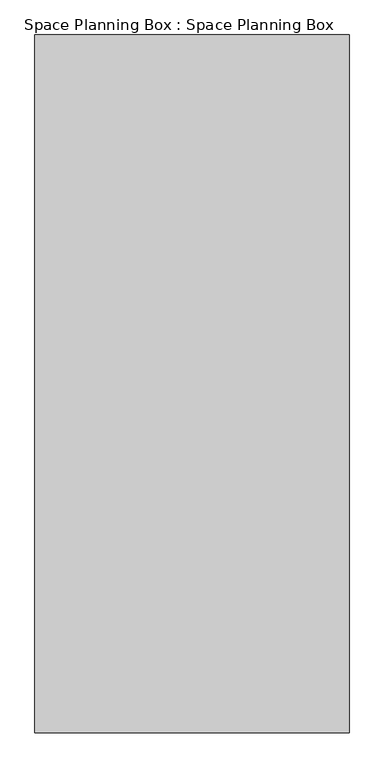
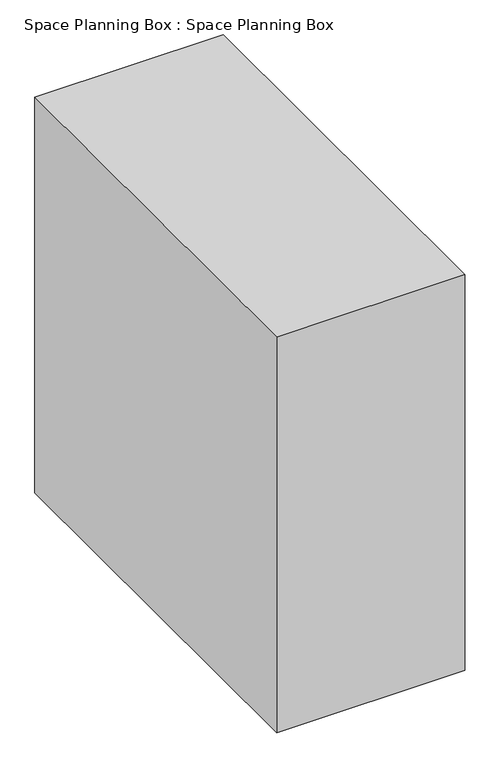
"""IFC4 building model written with IfcOpenShell, lengths in millimetres: proxy geometry, Space Planning Box : Space Planning Box."""

from ifc_helpers import new_model, si_unit, origin, origin_with_axes, place, context, project, spatial, polyline, outline, extrude, source, transform, mapped, element, save


def space_planning_box_space_planning_box_5634f436(model_context):
    return source(origin(), model_context, "Body", "SweptSolid", [
        extrude(outline(polyline([(1350.0, 3000.0), (1350.0, -3000.0), (-1350.0, -3000.0), (-1350.0, 3000.0), (1350.0, 3000.0)])), origin_with_axes(), (0.0, 0.0, 1.0), 6000.0),
    ])


if __name__ == "__main__":
    model = new_model("IFC4")
    model_context = context("Model", 3, world=origin())
    ifc_project = project(units=[si_unit("LENGTHUNIT", "METRE", prefix="MILLI")], contexts=[model_context])
    site = spatial("IfcSite", under=ifc_project)
    building = spatial("IfcBuilding", under=site)
    placement = place(None, origin())
    space_planning_box_space_planning_box_shape = space_planning_box_space_planning_box_5634f436(model_context)
    element("IfcBuildingElementProxy", 1, Name="Space Planning Box : Space Planning Box", ObjectType="Space Planning Box : Space Planning Box", at=placement, inside=building, context=model_context, shape_type="MappedRepresentation", body=[
        mapped(space_planning_box_space_planning_box_shape, transform((0.0, 0.0, 0.0), x_axis=(1.0, 0.0, 0.0), y_axis=(0.0, 1.0, 0.0), z_axis=(0.0, 0.0, 1.0))),
    ])
    save(model, "model.ifc")

# Revit data of these elements
# Type "Space Planning Box : Space Planning Box"
#   Type Comments = "..."
#   Room Name [instance default] = "?"
#   Assembly Code = "..."
#   Width [instance default] = 1524 mm
#   Program Area [instance default] = 0 m²
#   Length [instance default] = 1524 mm
#   Height [instance default] = 1524 mm
#   Area [instance default] = 2.32258 m²
#   Fill Color [instance default] = Cyan
#   Default Elevation = 0
# Element 1 (IfcBuildingElementProxy, "Space Planning Box : Space Planning Box")
#   Room Name = "Duct Shaft"
#   Width = 2700 mm
#   Program Area = 16.2 m²
#   Length = 6000 mm
#   Height = 6000 mm
#   Area = 16.2 m²
#   Fill Color = Pink
#   Materials on its faces: "Pink"
# Materials
#   "Cyan": class "Generic", colour RGB 0 255 255, transparency 0.2, Cost = 0
#   "Pink": class "Generic", colour RGB 255 105 180, transparency 0.2, Cost = 0
